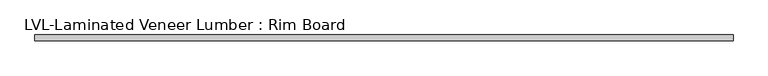
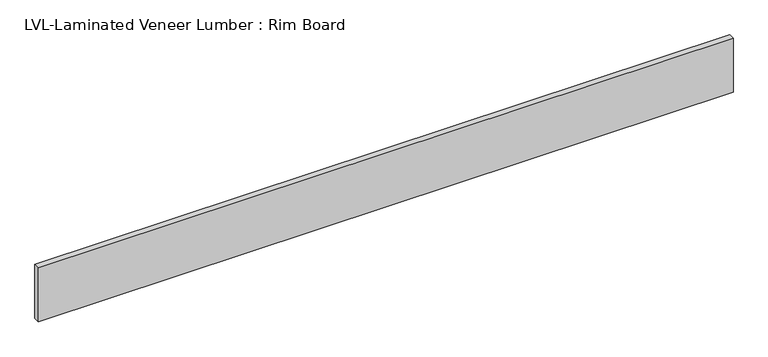
"""IFC4 building model written with IfcOpenShell, lengths in millimetres: beam geometry, LVL-Laminated Veneer Lumber : Rim Board."""

from ifc_helpers import new_model, si_unit, frame, origin, place, context, project, spatial, polyline, outline, extrude, source, transform, mapped, element, save


def lvl_laminated_veneer_lumber_rim_board_585cc746(model_context):
    return source(origin(), model_context, "Body", "SweptSolid", [
        extrude(outline(polyline([(1858.9625, 15.875), (1858.9625, -15.875), (-1827.2125, -15.875), (-1827.2125, 15.875), (1858.9625, 15.875)])), frame((0.0, 0.0, -150.8125), z_axis=(0.0, 0.0, 1.0), x_axis=(1.0, 0.0, 0.0)), (0.0, 0.0, 1.0), 301.625),
    ])


if __name__ == "__main__":
    model = new_model("IFC4")
    model_context = context("Model", 3, world=origin())
    ifc_project = project(units=[si_unit("LENGTHUNIT", "METRE", prefix="MILLI")], contexts=[model_context])
    site = spatial("IfcSite", under=ifc_project)
    building = spatial("IfcBuilding", under=site)
    placement = place(None, origin())
    lvl_laminated_veneer_lumber_rim_board_shape = lvl_laminated_veneer_lumber_rim_board_585cc746(model_context)
    element("IfcBeam", 1, ObjectType="LVL-Laminated Veneer Lumber : Rim Board", at=placement, inside=building, context=model_context, shape_type="MappedRepresentation", body=[
        mapped(lvl_laminated_veneer_lumber_rim_board_shape, transform((0.0, 0.0, 0.0), x_axis=(1.0, 0.0, 0.0), y_axis=(0.0, 1.0, 0.0), z_axis=(0.0, 0.0, 1.0))),
    ])
    save(model, "model.ifc")

# Revit data of these elements
# Type "LVL-Laminated Veneer Lumber : Rim Board"
#   Assembly Code = "B10"
#   Cost = 4.6
#   Length [instance default] = 5' - 0"
#   b = 0' - 1 1/4"
#   d = 0' - 11 7/8"
#   Structural Material [instance default] = Softwood, Lumber
# Element 1 (IfcBeam, "LVL-Laminated Veneer Lumber : Rim Board")
#   Structural Material = Douglas Fir #2
#   Materials on its faces: "Douglas Fir #2"
# Materials
#   "Softwood, Lumber": class "Wood", colour RGB 223 192 134, transparency 0, Description = "Pinus Echinata", Cost = 0
#   "Douglas Fir #2": class "Wood", colour RGB 223 192 134, transparency 0, Description = "Pinus Echinata", Cost = 0
